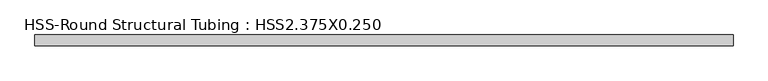
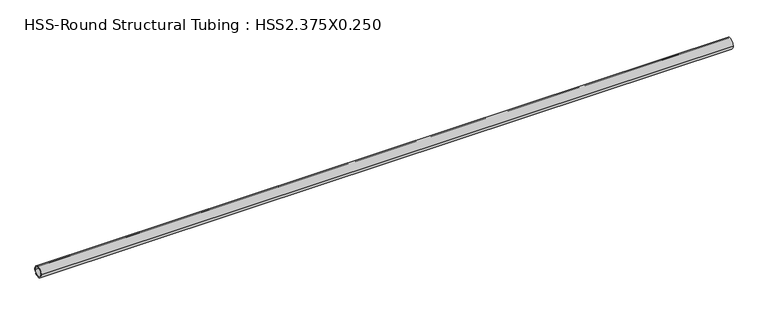
"""IFC4 building model written with IfcOpenShell, lengths in millimetres: beam geometry, HSS-Round Structural Tubing : HSS2.375X0.250."""

from ifc_helpers import new_model, si_unit, point, frame, origin, origin_2d, place, context, project, spatial, circle_curve, trimmed, segment, composite_curve, outline, extrude, source, transform, mapped, element, save


def hss_round_structural_tubing_hss2_375x0_250_b1115965(model_context):
    return source(origin(), model_context, "Body", "SweptSolid", [
        extrude(outline(composite_curve([segment(trimmed(circle_curve(origin_2d(), 30.1625), [point((-30.1625, 0.0))], [point((30.1625, 0.0))], False, "CARTESIAN"), True, "CONTINUOUS"), segment(trimmed(circle_curve(origin_2d(), 30.1625), [point((30.1625, 0.0))], [point((-30.1625, 0.0))], False, "CARTESIAN"), True, "CONTINUOUS")], self_intersect=False), holes=[composite_curve([segment(trimmed(circle_curve(origin_2d(), 24.2443), [point((24.2443, 0.0))], [point((-24.2443, 0.0))], True, "CARTESIAN"), True, "CONTINUOUS"), segment(trimmed(circle_curve(origin_2d(), 24.2443), [point((-24.2443, 0.0))], [point((24.2443, 0.0))], True, "CARTESIAN"), True, "CONTINUOUS")], self_intersect=False)]), frame((-1936.75, 0.0, 0.0), z_axis=(1.0, 0.0, 0.0), x_axis=(0.0, 1.0, 0.0)), (0.0, 0.0, 1.0), 3873.5),
    ])


if __name__ == "__main__":
    model = new_model("IFC4")
    model_context = context("Model", 3, world=origin())
    ifc_project = project(units=[si_unit("LENGTHUNIT", "METRE", prefix="MILLI")], contexts=[model_context])
    site = spatial("IfcSite", under=ifc_project)
    building = spatial("IfcBuilding", under=site)
    placement = place(None, origin())
    hss_round_structural_tubing_hss2_375x0_250_shape = hss_round_structural_tubing_hss2_375x0_250_b1115965(model_context)
    element("IfcBeam", 1, ObjectType="HSS-Round Structural Tubing : HSS2.375X0.250", at=placement, inside=building, context=model_context, shape_type="MappedRepresentation", body=[
        mapped(hss_round_structural_tubing_hss2_375x0_250_shape, transform((0.0, 0.0, 0.0), x_axis=(1.0, 0.0, 0.0), y_axis=(0.0, 1.0, 0.0), z_axis=(0.0, 0.0, 1.0))),
    ])
    save(model, "model.ifc")

# Revit data of these elements
# Type "HSS-Round Structural Tubing : HSS2.375X0.250"
#   Assembly Code = "B10"
#   t = 0' - 0.233"
#   W = 5.68
#   Length [instance default] = 5' - 0"
#   OD = 0' - 2 3/8"
#   A = 0.0109028 SF
#   Structural Material [instance default] = Steel ASTM A500, Grade B, Round
# Element 1 (IfcBeam, "HSS-Round Structural Tubing : HSS2.375X0.250")
#   Structural Material = Aluminum
#   Materials on its faces: "Aluminum"
# Materials
#   "Steel ASTM A500, Grade B, Round": class "Metal", colour RGB 199 199 199, transparency 0, Description = "Carbon steel", Cost = 0
#   "Aluminum": class "Metal", colour RGB 247 247 247, transparency 0, Description = "Aluminum 6061", Cost = 0
